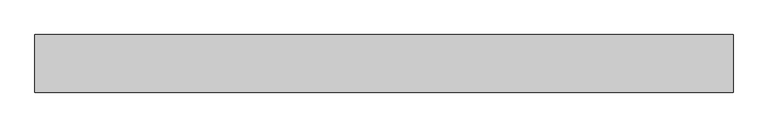
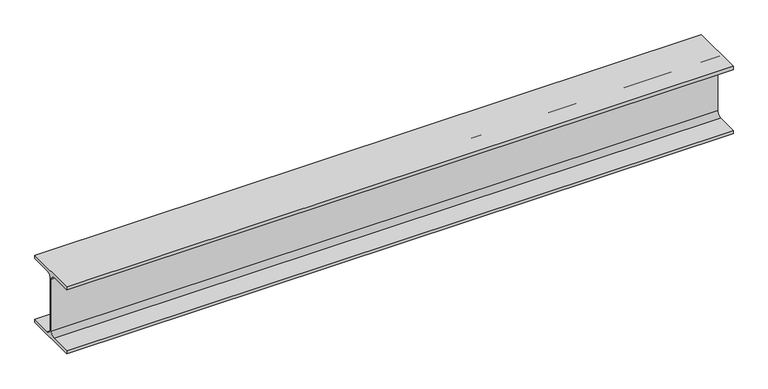
"""IFC4 building model written with IfcOpenShell, lengths in millimetres: beam geometry, 0912_Steel Framing_H-KSD3502 : H_SB_ASB_H-194x150x6x9."""

from ifc_helpers import new_model, si_unit, point, frame, frame_2d, origin, place, context, project, spatial, polyline, circle_curve, trimmed, segment, composite_curve, outline, extrude, source, transform, mapped, element, save


def beam_b1e6920e(model_context):
    return source(origin(), model_context, "Body", "SweptSolid", [
        extrude(outline(composite_curve([segment(polyline([(-75.0, -88.0), (-16.0, -88.0)]), True, "CONTINUOUS"), segment(trimmed(circle_curve(frame_2d((-16.0, -75.0)), 13.0), [point((-16.0, -88.0))], [point((-3.0, -75.0))], True, "CARTESIAN"), True, "CONTINUOUS"), segment(polyline([(-3.0, -75.0), (-3.0, 75.0)]), True, "CONTINUOUS"), segment(trimmed(circle_curve(frame_2d((-16.0, 75.0)), 13.0), [point((-3.0, 75.0))], [point((-16.0, 88.0))], True, "CARTESIAN"), True, "CONTINUOUS"), segment(polyline([(-16.0, 88.0), (-75.0, 88.0), (-75.0, 97.0), (75.0, 97.0), (75.0, 88.0), (16.0, 88.0)]), True, "CONTINUOUS"), segment(trimmed(circle_curve(frame_2d((16.0, 75.0)), 13.0), [point((16.0, 88.0))], [point((3.0, 75.0))], True, "CARTESIAN"), True, "CONTINUOUS"), segment(polyline([(3.0, 75.0), (3.0, -75.0)]), True, "CONTINUOUS"), segment(trimmed(circle_curve(frame_2d((16.0, -75.0)), 13.0), [point((3.0, -75.0))], [point((16.0, -88.0))], True, "CARTESIAN"), True, "CONTINUOUS"), segment(polyline([(16.0, -88.0), (75.0, -88.0), (75.0, -97.0), (-75.0, -97.0), (-75.0, -88.0)]), True, "CONTINUOUS")], self_intersect=False)), frame((-908.9645727, 0.0, 0.0), z_axis=(1.0, 0.0, 0.0), x_axis=(0.0, 1.0, 0.0)), (0.0, 0.0, 1.0), 1817.9291455),
    ])


if __name__ == "__main__":
    model = new_model("IFC4")
    model_context = context("Model", 3, world=origin())
    ifc_project = project(units=[si_unit("LENGTHUNIT", "METRE", prefix="MILLI")], contexts=[model_context])
    site = spatial("IfcSite", under=ifc_project)
    building = spatial("IfcBuilding", under=site)
    placement = place(None, origin())
    beam_shape = beam_b1e6920e(model_context)
    element("IfcBeam", 1, ObjectType="0912_Steel Framing_H-KSD3502 : H_SB_ASB_H-194x150x6x9", at=placement, inside=building, context=model_context, shape_type="MappedRepresentation", body=[
        mapped(beam_shape, transform((0.0, 0.0, 0.0), x_axis=(1.0, 0.0, 0.0), y_axis=(0.0, 1.0, 0.0), z_axis=(0.0, 0.0, 1.0))),
    ])
    save(model, "model.ifc")

# Revit data of these elements
# Type "0912_Steel Framing_H-KSD3502 : H_SB_ASB_H-194x150x6x9"
#   H_WM Code_1 = "S01AA002-00001 | Main Steel Structure Fabrication Work | Shelter/Building | Medium Steel - Standard (90KG/M>Weight≥30KG/M) | Material: (   )"
#   H_WM Code_2 = "S03AA028-00001 | Main Steel Structure Erection Work | Shelter/Building | Medium Steel (90KG/M>Weight≥30KG/M) | Material: (   )"
#   H_WM Code_3 = "S01AA010-00001 | Main Steel Structure Fabrication Work | Shelter/Building | Steel Painting/Coating | for Non-Fireproofed Steel Surface, Surface Preparation, Primer, Second & Final Coat | Material: (   )"
#   H_Q'ty Cal Type Tag = "SB-Q2"
#   Width = 15.0 cm
#   Web Thickness = 0.6 cm
#   Web Fillet = 1.3 cm
#   Warping Constant = 43316.0 cm⁶
#   W = 0
#   Torsional Moment of Inertia = 8.622 cm⁴
#   Section Area = 39.01 cm²
#   Plastic Modulus weak axis = 104.0 cm³
#   Plastic Modulus strong axis = 309.0 cm³
#   Perimeter = 0.95 m²/m
#   Nominal Weight = 30.60 kgf/m
#   Moment of Inertia weak axis = 507.00 cm⁴
#   Moment of Inertia strong axis = 2690.00 cm⁴
#   Height = 19.4 cm
#   Flange Thickness = 0.9 cm
#   Elastic Modulus weak axis = 67.6 cm³
#   Elastic Modulus strong axis = 277.0 cm³
#   Centroid Vertical = 9.7 cm
#   Centroid Horizontal = 7.5 cm
#   Ix = 26900000
#   Length [instance default] = 1.5240 m
#   Zx = 309000
#   b = 0.1500 m
#   h = 0.1940 m
#   r = 0.0130 m
#   s = 0.0060 m
#   t = 0.0090 m
#   A = 0.003901 m²
#   Structural Material [instance default] = Steel, 45-345
#   Assembly Code = ""
# Element 1 (IfcBeam, "0912_Steel Framing_H-KSD3502 : H_SB_ASB_H-194x150x6x9")
#   Structural Material = none
# Materials
#   "Steel, 45-345": class "Metal", colour RGB 189 187 185, transparency 0, Description = "Steel 345 MPa", Cost = 0
